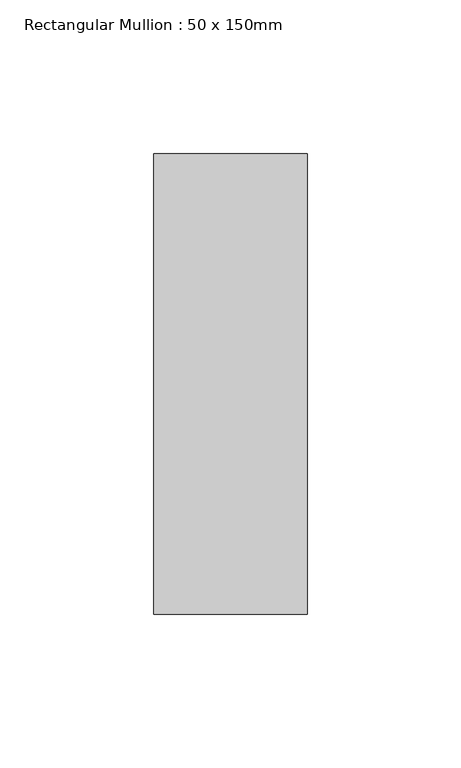
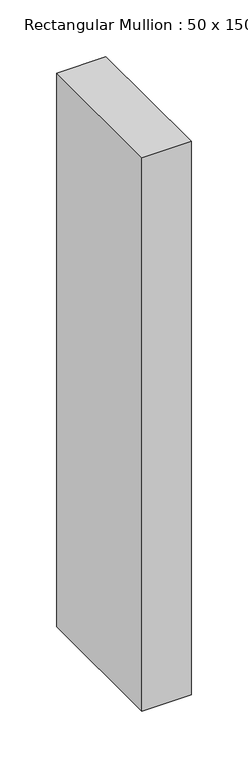
"""IFC4 building model written with IfcOpenShell, lengths in millimetres: member geometry, Rectangular Mullion : 50 x 150mm."""

from ifc_helpers import new_model, si_unit, frame, origin, place, context, project, spatial, polyline, outline, extrude, source, transform, mapped, element, save


def rectangular_mullion_50_x_150mm_b23e394a(model_context):
    return source(origin(), model_context, "Body", "SweptSolid", [
        extrude(outline(polyline([(0.0, 75.0), (0.0, -75.0), (-50.0, -75.0), (-50.0, 75.0), (0.0, 75.0)])), frame((0.0, 0.0, -595.0), z_axis=(0.0, 0.0, 1.0), x_axis=(1.0, 0.0, 0.0)), (0.0, 0.0, 1.0), 595.0),
    ])


if __name__ == "__main__":
    model = new_model("IFC4")
    model_context = context("Model", 3, world=origin())
    ifc_project = project(units=[si_unit("LENGTHUNIT", "METRE", prefix="MILLI")], contexts=[model_context])
    site = spatial("IfcSite", under=ifc_project)
    building = spatial("IfcBuilding", under=site)
    placement = place(None, origin())
    rectangular_mullion_50_x_150mm_shape = rectangular_mullion_50_x_150mm_b23e394a(model_context)
    element("IfcMember", 1, ObjectType="Rectangular Mullion : 50 x 150mm", at=placement, inside=building, context=model_context, shape_type="MappedRepresentation", body=[
        mapped(rectangular_mullion_50_x_150mm_shape, transform((0.0, 0.0, 0.0), x_axis=(1.0, 0.0, 0.0), y_axis=(0.0, 1.0, 0.0), z_axis=(0.0, 0.0, 1.0))),
    ])
    save(model, "model.ifc")

# Revit data of these elements
# Type "Rectangular Mullion : 50 x 150mm"
#   built-in parameter 1007304 = 0.492126 (stored number, unit not read)
#   built-in parameter 1007301 = 0.082021 (stored number, unit not read)
#   built-in parameter 1007300 = 0.082021 (stored number, unit not read)
# Element 1 (IfcMember, "Rectangular Mullion : 50 x 150mm")
#   Materials on its faces: "Metal - Aluminium"
# Materials
#   "Metal - Aluminium": class "Metal", colour RGB 247 247 247, transparency 0
